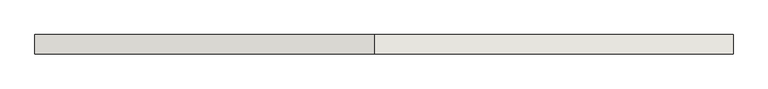
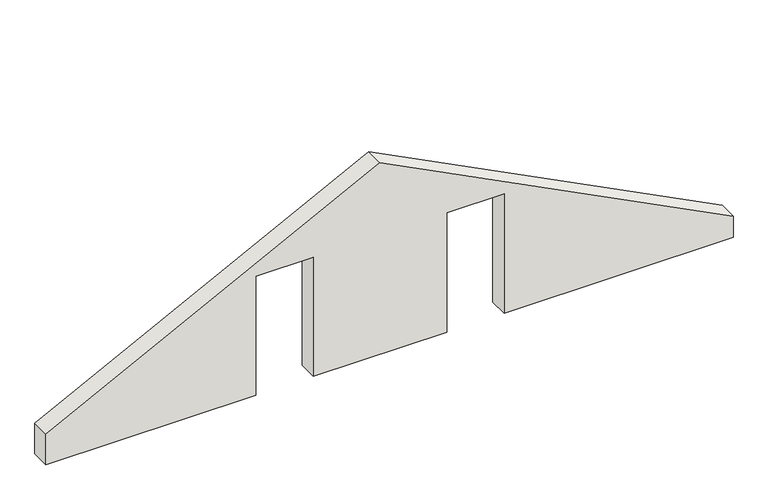
"""IFC4 building model written with IfcOpenShell, lengths in millimetres: wall geometry, 0_3d."""

from ifc_helpers import new_model, si_unit, frame, origin, place, context, project, spatial, polyline, outline, extrude, source, transform, mapped, element, save


def wall_d46ac6a4(model_context):
    return source(origin(), model_context, "Body", "SweptSolid", [
        extrude(outline(polyline([(2500.0, 5295.0), (0.0, 5295.0), (0.0, 7945.0), (2500.0, 7945.0), (2500.0, 9080.0), (0.0, 9080.0), (0.0, 13620.0), (445.0, 13620.0), (4011.6781465, 6620.0), (638.6196708, 0.0), (0.0, 0.0), (0.0, 4160.0), (2500.0, 4160.0), (2500.0, 5295.0)])), frame((0.0, 0.0, 0.0), z_axis=(0.0, 1.0, 0.0), x_axis=(0.0, 0.0, 1.0)), (0.0, 0.0, 1.0), 380.0),
    ])


if __name__ == "__main__":
    model = new_model("IFC4")
    model_context = context("Model", 3, world=origin())
    ifc_project = project(units=[si_unit("LENGTHUNIT", "METRE", prefix="MILLI")], contexts=[model_context])
    site = spatial("IfcSite", under=ifc_project)
    building = spatial("IfcBuilding", under=site)
    placement = place(None, origin())
    wall_shape = wall_d46ac6a4(model_context)
    element("IfcWall", 1, ObjectType="0_3d", at=placement, inside=building, context=model_context, shape_type="MappedRepresentation", body=[
        mapped(wall_shape, transform((0.0, 0.0, 0.0), x_axis=(1.0, 0.0, 0.0), y_axis=(0.0, 1.0, 0.0), z_axis=(0.0, 0.0, 1.0))),
    ])
    save(model, "model.ifc")

# Revit data of these elements
# Element 1 (IfcWall, "0_3d")
#   Materials on its faces: "holzschalung"
# Materials
#   "holzschalung": class "Unassigned", colour RGB 128 128 128, transparency 0
